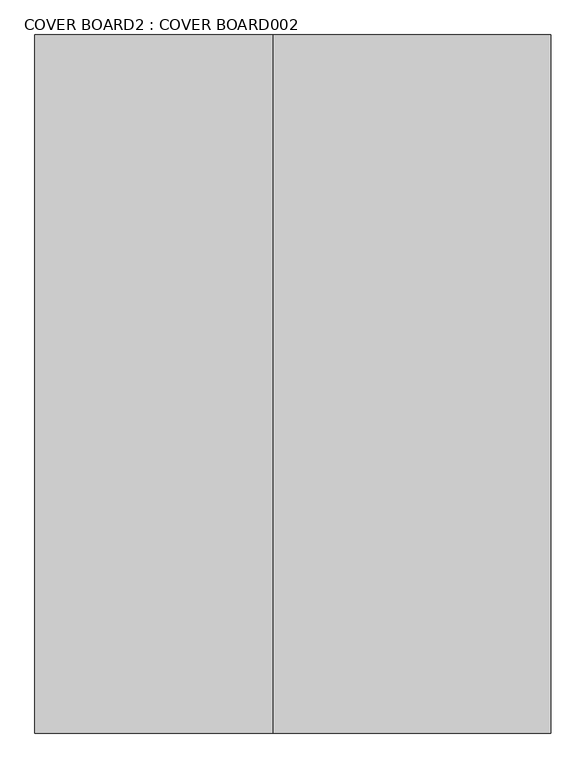
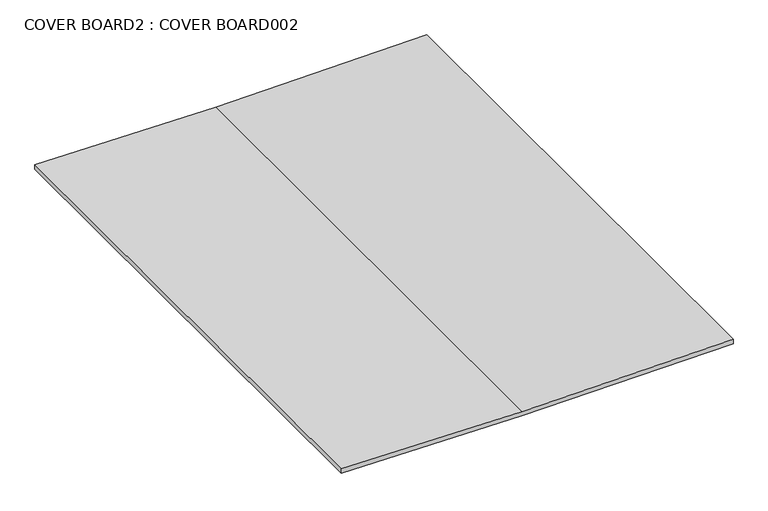
"""IFC4 building model written with IfcOpenShell, lengths in millimetres: proxy geometry, COVER BOARD2 : COVER BOARD002."""

import ifcopenshell
import ifcopenshell.guid

model = None  # the IFC model being written
_history = None  # IfcOwnerHistory: only IFC2X3 demands one
_inside = {}  # id of a spatial element -> (the spatial element, [elements in it])
_under = {}  # id of a project, library or spatial element -> (it, [spatial elements below it])
_declared = {}  # id of a project -> (the project, [libraries it declares])
_typed = {}  # id of a type object -> (the type object, [elements of that type])
_made_of = {}  # id of a material, layer set ... -> (it, [elements and type objects made of it])


def new_model(schema):
    """Start an empty IFC model of exactly this schema.

    Asked for "IFC4X3", IfcOpenShell would pick the latest addendum, in which some entities
    have other attributes; the version numbers below select the first issue.
    IFC2X3 requires an IfcOwnerHistory on every rooted entity: one is made here for all.
    """
    global model, _history
    if schema == "IFC4X3":
        model = ifcopenshell.file(schema_version=(4, 3, 0, 0))
    else:
        model = ifcopenshell.file(schema=schema)
    _inside.clear()
    _under.clear()
    _declared.clear()
    _typed.clear()
    _made_of.clear()
    _history = None
    if model.schema == "IFC2X3":
        org = make("IfcOrganization", Name="unknown")
        user = make(
            "IfcPersonAndOrganization",
            ThePerson=make("IfcPerson", FamilyName="unknown"),
            TheOrganization=org,
        )
        app = make(
            "IfcApplication",
            ApplicationDeveloper=org,
            Version="unknown",
            ApplicationFullName="unknown",
            ApplicationIdentifier="unknown",
        )
        _history = make(
            "IfcOwnerHistory",
            OwningUser=user,
            OwningApplication=app,
            ChangeAction="ADDED",
            CreationDate=0,
        )
    return model


def make(cls, **values):
    """One entity of the class cls with the attributes given. An attribute that is None is left unset."""
    return model.create_entity(
        cls, **{name: value for name, value in values.items() if value is not None}
    )


def rooted(cls, **values):
    """An entity with a GlobalId (a new one), such as an element, a storey or a relation."""
    return make(cls, GlobalId=ifcopenshell.guid.new(), OwnerHistory=_history, **values)


def si_unit(unit_type, name, prefix=None):
    """IfcSIUnit, for example si_unit("LENGTHUNIT", "METRE", prefix="MILLI")."""
    return make("IfcSIUnit", UnitType=unit_type, Prefix=prefix, Name=name)


def assignment(units):
    """IfcUnitAssignment: the units of a project."""
    return None if units is None else make("IfcUnitAssignment", Units=units)


def point(xyz):
    """IfcCartesianPoint."""
    return None if xyz is None else make("IfcCartesianPoint", Coordinates=xyz)


def direction(xyz):
    """IfcDirection."""
    return None if xyz is None else make("IfcDirection", DirectionRatios=xyz)


def frame(location, z_axis=None, x_axis=None):
    """IfcAxis2Placement3D, a coordinate frame: its origin and axes. An axis left out is left unset."""
    return make(
        "IfcAxis2Placement3D",
        Location=point(location),
        Axis=direction(z_axis),
        RefDirection=direction(x_axis),
    )


def origin():
    """The frame at (0, 0, 0) with its axes left unset."""
    return frame((0.0, 0.0, 0.0))


def place(relative_to, where):
    """IfcLocalPlacement: puts the frame where relative to a parent placement (None: the world)."""
    return make(
        "IfcLocalPlacement", PlacementRelTo=relative_to, RelativePlacement=where
    )


def context(
    kind, dimensions, precision=None, world=None, true_north=None, identifier=None
):
    """IfcGeometricRepresentationContext, for example the 3D "Model" context."""
    return make(
        "IfcGeometricRepresentationContext",
        ContextIdentifier=identifier,
        ContextType=kind,
        CoordinateSpaceDimension=dimensions,
        Precision=precision,
        WorldCoordinateSystem=world,
        TrueNorth=true_north,
    )


def project(units=None, contexts=None):
    """IfcProject with its units and contexts."""
    return rooted(
        "IfcProject",
        Name="project",
        RepresentationContexts=contexts,
        UnitsInContext=assignment(units),
    )


def spatial(cls, under=None, at=None, **own):
    """A site, building, storey or space (cls), placed at a placement, below another one or the project."""
    s = rooted(cls, ObjectPlacement=at, **own)
    if under is not None:
        _under.setdefault(under.id(), (under, []))[1].append(s)
    return s


def polyline(points):
    """IfcPolyline through the points."""
    return make("IfcPolyline", Points=[point(p) for p in points])


def outline(outer, holes=None, kind="AREA"):
    """IfcArbitraryClosedProfileDef: a profile drawn as a closed curve; with holes, ...WithVoids."""
    if holes is None:
        return make("IfcArbitraryClosedProfileDef", ProfileType=kind, OuterCurve=outer)
    return make(
        "IfcArbitraryProfileDefWithVoids",
        ProfileType=kind,
        OuterCurve=outer,
        InnerCurves=holes,
    )


def extrude(swept, where, along, depth):
    """IfcExtrudedAreaSolid: the profile swept, set in the frame where, extruded along a direction by depth."""
    return make(
        "IfcExtrudedAreaSolid",
        SweptArea=swept,
        Position=where,
        ExtrudedDirection=direction(along),
        Depth=depth,
    )


def shape(context_of_items, identifier, shape_type, items):
    """IfcShapeRepresentation: the items that make up one representation, for example the "Body"."""
    return make(
        "IfcShapeRepresentation",
        ContextOfItems=context_of_items,
        RepresentationIdentifier=identifier,
        RepresentationType=shape_type,
        Items=items,
    )


def source(mapping_origin, context_of_items, identifier, shape_type, items):
    """IfcRepresentationMap: a shape defined once, which mapped items show again and again."""
    return make(
        "IfcRepresentationMap",
        MappingOrigin=mapping_origin,
        MappedRepresentation=shape(context_of_items, identifier, shape_type, items),
    )


def transform(
    local_origin,
    x_axis=None,
    y_axis=None,
    z_axis=None,
    scale=None,
    scale2=None,
    scale3=None,
    uniform=True,
):
    """IfcCartesianTransformationOperator3D, or its non-uniform kind. x_axis, y_axis, z_axis: its Axis1, 2, 3."""
    if uniform:
        return make(
            "IfcCartesianTransformationOperator3D",
            Axis1=direction(x_axis),
            Axis2=direction(y_axis),
            LocalOrigin=point(local_origin),
            Scale=scale,
            Axis3=direction(z_axis),
        )
    return make(
        "IfcCartesianTransformationOperator3DnonUniform",
        Axis1=direction(x_axis),
        Axis2=direction(y_axis),
        LocalOrigin=point(local_origin),
        Scale=scale,
        Axis3=direction(z_axis),
        Scale2=scale2,
        Scale3=scale3,
    )


def mapped(mapping_source, mapping_target):
    """IfcMappedItem: shows the shape of a source again, moved by a transform."""
    return make(
        "IfcMappedItem", MappingSource=mapping_source, MappingTarget=mapping_target
    )


def made_of(thing, what):
    """Note that an element or type object is made of a material, layer set ...; save() writes the relation."""
    if what is not None:
        _made_of.setdefault(what.id(), (what, []))[1].append(thing)
    return thing


def element(
    cls,
    number,
    at=None,
    inside=None,
    cuts=None,
    type_object=None,
    material=None,
    context=None,
    identifier="Body",
    shape_type=None,
    held_by="IfcProductDefinitionShape",
    body=None,
    shapes=None,
    **own,
):
    """One element of the class cls, such as IfcWall. Its Tag is "e" and its number.

    at: its placement. inside: the storey or other place that contains it. cuts: it is an
    opening in that element (IfcRelVoidsElement). A single representation is given by context,
    identifier, shape_type and body (its items); several are given by shapes. held_by: the class
    of the entity that holds the representations. save() writes the other relations.
    """
    e = rooted(cls, Tag="e%d" % number, ObjectPlacement=at, **own)
    if body is not None:
        shapes = [shape(context, identifier, shape_type, body)]
    if shapes is not None:
        e.Representation = make(held_by, Representations=shapes)
    if inside is not None:
        _inside.setdefault(inside.id(), (inside, []))[1].append(e)
    if cuts is not None:
        rooted(
            "IfcRelVoidsElement", RelatingBuildingElement=cuts, RelatedOpeningElement=e
        )
    if type_object is not None:
        _typed.setdefault(type_object.id(), (type_object, []))[1].append(e)
    return made_of(e, material)


def aggregate(whole, parts):
    """IfcRelAggregates: a whole, such as a stair, and the parts it consists of."""
    return rooted("IfcRelAggregates", RelatingObject=whole, RelatedObjects=parts)


def save(model, path):
    """Write the relations noted so far, then the file.

    IfcRelAggregates (storeys below a building ...), IfcRelContainedInSpatialStructure (elements
    in a storey), IfcRelDefinesByType, IfcRelAssociatesMaterial and IfcRelDeclares: one each for
    every whole, place, type object, material and project.
    """
    for whole, parts in _under.values():
        aggregate(whole, parts)
    for where, things in _inside.values():
        rooted(
            "IfcRelContainedInSpatialStructure",
            RelatedElements=things,
            RelatingStructure=where,
        )
    for kind, things in _typed.values():
        rooted("IfcRelDefinesByType", RelatedObjects=things, RelatingType=kind)
    for what, things in _made_of.values():
        rooted("IfcRelAssociatesMaterial", RelatedObjects=things, RelatingMaterial=what)
    for by, libraries in _declared.values():
        rooted("IfcRelDeclares", RelatingContext=by, RelatedDefinitions=libraries)
    model.write(path)


def cover_board2_cover_board002_e83da0d9(model_context):
    return source(origin(), model_context, "Body", "SweptSolid", [
        extrude(outline(polyline([(40228.1021556, -1886.5629484), (40237.9000089, -2567.3737014), (40220.5682898, -2567.3737014), (40210.7704365, -1886.5629484), (40220.5682898, -1090.0815411), (40237.9000089, -1090.0815411), (40228.1021556, -1886.5629484)])), frame((0.0, 1000.0, 0.0), z_axis=(0.0, 1.0, 0.0), x_axis=(0.0, 0.0, 1.0)), (0.0, 0.0, 1.0), 2000.0),
    ])


if __name__ == "__main__":
    model = new_model("IFC4")
    model_context = context("Model", 3, world=origin())
    ifc_project = project(units=[si_unit("LENGTHUNIT", "METRE", prefix="MILLI")], contexts=[model_context])
    site = spatial("IfcSite", under=ifc_project)
    building = spatial("IfcBuilding", under=site)
    placement = place(None, origin())
    cover_board2_cover_board002_shape = cover_board2_cover_board002_e83da0d9(model_context)
    element("IfcBuildingElementProxy", 1, Name="COVER BOARD2 : COVER BOARD002", ObjectType="COVER BOARD2 : COVER BOARD002", at=placement, inside=building, context=model_context, shape_type="MappedRepresentation", body=[
        mapped(cover_board2_cover_board002_shape, transform((0.0, 0.0, 0.0), x_axis=(1.0, 0.0, 0.0), y_axis=(0.0, 1.0, 0.0), z_axis=(0.0, 0.0, 1.0))),
    ])
    save(model, "model.ifc")

# Revit data of these elements
# Type "COVER BOARD2 : COVER BOARD002"
#   NameOverride = "COVER BOARD002"
# Element 1 (IfcBuildingElementProxy, "COVER BOARD2 : COVER BOARD002")
#   Materials on its faces: "CDX PLYWOOD - SEE STRUCTURAL DWGS"
# Materials
#   "CDX PLYWOOD - SEE STRUCTURAL DWGS": class "Unassigned", colour RGB 202 163 108, transparency 0, Cost = 0
